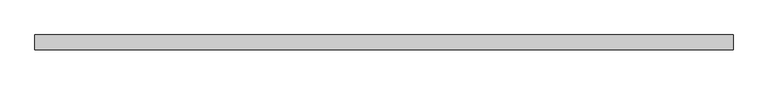
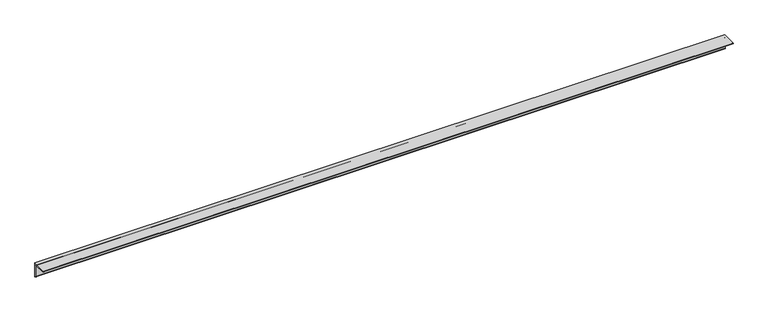
"""IFC4 building model written with IfcOpenShell, lengths in millimetres: member geometry, 0912_Steel Framing_L-KSD3502 : H_SB_AR_S03_L-130x130x12_HBR3."""

from ifc_helpers import new_model, si_unit, point, frame, frame_2d, origin, place, context, project, spatial, polyline, circle_curve, trimmed, segment, composite_curve, outline, extrude, source, transform, mapped, element, save


def member_fa0e1bc2(model_context):
    return source(origin(), model_context, "Body", "SweptSolid", [
        extrude(outline(composite_curve([segment(polyline([(36.4, 36.4), (36.4, -93.6)]), True, "CONTINUOUS"), segment(trimmed(circle_curve(frame_2d((36.4, -81.6)), 12.0), [point((36.4, -93.6))], [point((24.4, -81.6))], False, "CARTESIAN"), True, "CONTINUOUS"), segment(polyline([(24.4, -81.6), (24.4, 12.4)]), True, "CONTINUOUS"), segment(trimmed(circle_curve(frame_2d((12.4, 12.4)), 12.0), [point((24.4, 12.4))], [point((12.4, 24.4))], True, "CARTESIAN"), True, "CONTINUOUS"), segment(polyline([(12.4, 24.4), (-81.6, 24.4)]), True, "CONTINUOUS"), segment(trimmed(circle_curve(frame_2d((-81.6, 36.4)), 12.0), [point((-81.6, 24.4))], [point((-93.6, 36.4))], False, "CARTESIAN"), True, "CONTINUOUS"), segment(polyline([(-93.6, 36.4), (36.4, 36.4)]), True, "CONTINUOUS")], self_intersect=False)), frame((-3145.2559782, 0.0, 0.0), z_axis=(1.0, 0.0, 0.0), x_axis=(0.0, 1.0, 0.0)), (0.0, 0.0, 1.0), 6164.5036212),
    ])


if __name__ == "__main__":
    model = new_model("IFC4")
    model_context = context("Model", 3, world=origin())
    ifc_project = project(units=[si_unit("LENGTHUNIT", "METRE", prefix="MILLI")], contexts=[model_context])
    site = spatial("IfcSite", under=ifc_project)
    building = spatial("IfcBuilding", under=site)
    placement = place(None, origin())
    member_shape = member_fa0e1bc2(model_context)
    element("IfcMember", 1, ObjectType="0912_Steel Framing_L-KSD3502 : H_SB_AR_S03_L-130x130x12_HBR3", at=placement, inside=building, context=model_context, shape_type="MappedRepresentation", body=[
        mapped(member_shape, transform((0.0, 0.0, 0.0), x_axis=(1.0, 0.0, 0.0), y_axis=(0.0, 1.0, 0.0), z_axis=(0.0, 0.0, 1.0))),
    ])
    save(model, "model.ifc")

# Revit data of these elements
# Type "0912_Steel Framing_L-KSD3502 : H_SB_AR_S03_L-130x130x12_HBR3"
#   k = 25 mm
#   Perimeter = 0.52 m²/m
#   Nominal Weight = 23.40 kgf/m
#   Length [instance default] = 1000 mm
#   b = 130 mm
#   d = 130 mm
#   t = 12 mm
#   x = 36.4 mm
#   y = 36.4 mm
#   A = 2976.00 m²
#   Structural Material [instance default] = Steel, 45-345
# Element 1 (IfcMember, "0912_Steel Framing_L-KSD3502 : H_SB_AR_S03_L-130x130x12_HBR3")
#   Structural Material = Steel ASTM A36
#   Materials on its faces: "Steel ASTM A36"
# Materials
#   "Steel, 45-345": class "Metal", colour RGB 189 187 185, transparency 0, Description = "Steel 345 MPa", Cost = 0
#   "Steel ASTM A36": class "Metal", colour RGB 199 199 199, transparency 0, Description = "Structural steel, ASTM A36 Grade B, mill finish", Cost = 0
